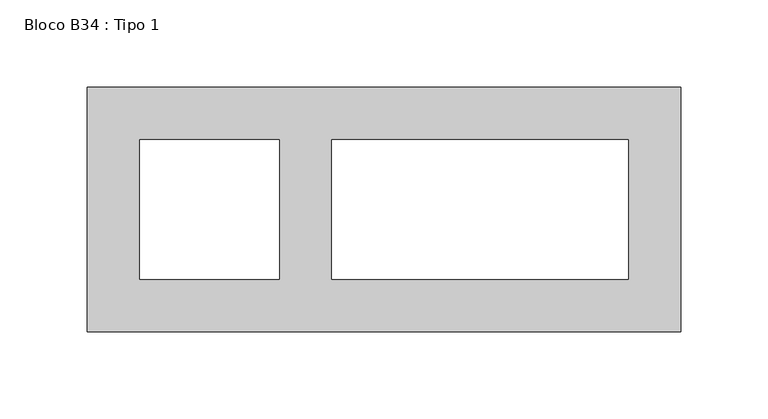
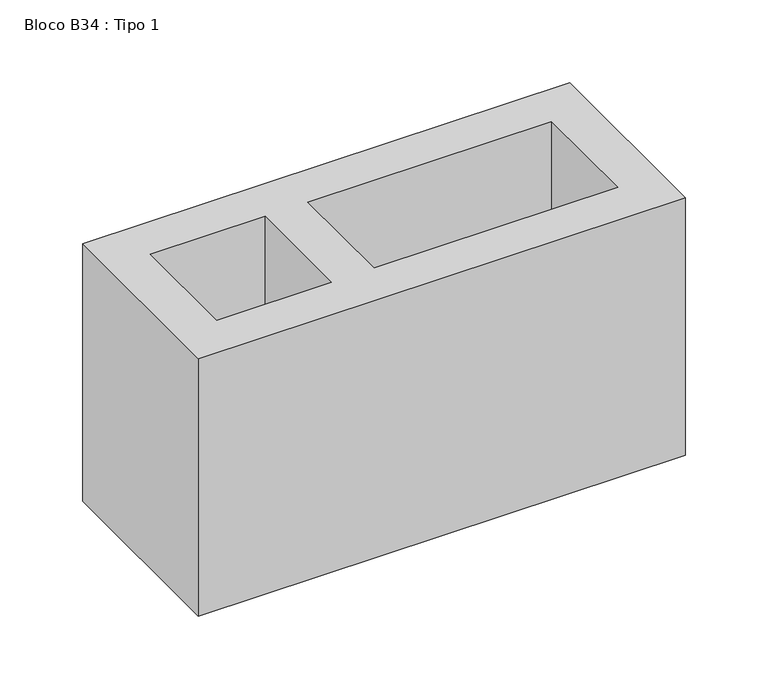
"""IFC4 building model written with IfcOpenShell, lengths in millimetres: proxy geometry, Bloco B34 : Tipo 1."""

from ifc_helpers import new_model, si_unit, origin, origin_with_axes, place, context, project, spatial, polyline, outline, extrude, source, transform, mapped, element, save


def bloco_b34_tipo_1_da18a2fe(model_context):
    return source(origin(), model_context, "Body", "SweptSolid", [
        extrude(outline(polyline([(340.0, 140.0), (340.0, 0.0), (0.0, 0.0), (0.0, 140.0), (340.0, 140.0)]), holes=[polyline([(110.0, 110.0), (30.0, 110.0), (30.0, 30.0), (110.0, 30.0), (110.0, 110.0)]), polyline([(140.0, 110.0), (140.0, 30.0), (310.0, 30.0), (310.0, 110.0), (140.0, 110.0)])]), origin_with_axes(), (0.0, 0.0, 1.0), 190.0),
    ])


if __name__ == "__main__":
    model = new_model("IFC4")
    model_context = context("Model", 3, world=origin())
    ifc_project = project(units=[si_unit("LENGTHUNIT", "METRE", prefix="MILLI")], contexts=[model_context])
    site = spatial("IfcSite", under=ifc_project)
    building = spatial("IfcBuilding", under=site)
    placement = place(None, origin())
    bloco_b34_tipo_1_shape = bloco_b34_tipo_1_da18a2fe(model_context)
    element("IfcBuildingElementProxy", 1, Name="Bloco B34 : Tipo 1", ObjectType="Bloco B34 : Tipo 1", at=placement, inside=building, context=model_context, shape_type="MappedRepresentation", body=[
        mapped(bloco_b34_tipo_1_shape, transform((0.0, 0.0, 0.0), x_axis=(1.0, 0.0, 0.0), y_axis=(0.0, 1.0, 0.0), z_axis=(0.0, 0.0, 1.0))),
    ])
    save(model, "model.ifc")

# Revit data of these elements
# Type "Bloco B34 : Tipo 1"
#   SINAPI = ""
#   Assembly Code = ""
